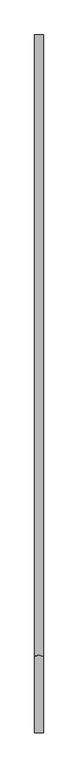
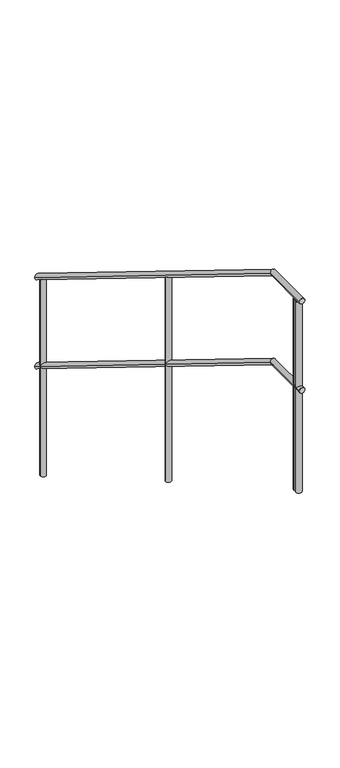
"""IFC4 building model written with IfcOpenShell, lengths in millimetres: railing geometry."""

from ifc_helpers import new_model, si_unit, point, frame, frame_2d, origin, place, context, project, spatial, circle_curve, ellipse_curve, trimmed, segment, composite_curve, outline, extrude, source, transform, mapped, element, save
from ifc_brep_helpers import plane_surface, cylinder_surface, advanced_brep


def railing_1ddb9561(model_context):
    return source(origin(), model_context, "Body", "SolidModel", [
        advanced_brep(
        [(-2206.0, 15342.7934796, -450.9609787), (-2176.0, 15342.7934796, -450.9609787), (-2176.0, 13178.5366941, 885.0), (-2206.0, 13178.5366941, 885.0), (-2206.0, 12912.7934796, 885.0), (-2176.0, 12912.7934796, 885.0)],
        [
            (0, 1, ellipse_curve(frame((-2191.0, 15342.7934796, -450.9609787), z_axis=(0.0, 1.0, 0.0), x_axis=(0.0, 0.0, -1.0)), 17.6276454, 15.0)),
            (1, 0, ellipse_curve(frame((-2191.0, 15342.7934796, -450.9609787), z_axis=(0.0, 1.0, 0.0), x_axis=(0.0, 0.0, -1.0)), 17.6276454, 15.0)),
            (1, 2),
            (2, 3, ellipse_curve(frame((-2191.0, 13178.5366941, 885.0), z_axis=(0.0, 0.9620125025549409, -0.27300539358770887), x_axis=(0.0, -0.27300539358770864, -0.962012502554941)), 15.5923129, 15.0)),
            (3, 0),
            (3, 2, ellipse_curve(frame((-2191.0, 13178.5366941, 885.0), z_axis=(0.0, 0.9620125025549409, -0.27300539358770887), x_axis=(0.0, -0.27300539358770864, -0.962012502554941)), 15.5923129, 15.0)),
            (4, 5, circle_curve(frame((-2191.0, 12912.7934796, 885.0), z_axis=(0.0, -1.0, 0.0), x_axis=(1.0, 0.0, 0.0)), 15.0)),
            (5, 4, circle_curve(frame((-2191.0, 12912.7934796, 885.0), z_axis=(0.0, -1.0, 0.0), x_axis=(1.0, 0.0, 0.0)), 15.0)),
            (2, 5),
            (4, 3),
        ],
        [
            plane_surface(frame((-2191.0, 15342.7934796, -433.3333333), z_axis=(0.0, 1.0, 0.0), x_axis=(0.0, 0.0, -1.0))),
            cylinder_surface(frame((-2191.0, 15334.9144415, -446.097375), z_axis=(0.0, 0.8509361101440404, -0.5252692037926169), x_axis=(1.0, 0.0, 0.0)), 15.0),
            plane_surface(frame((-2191.0, 12912.7934796, 900.0), z_axis=(0.0, -1.0, 0.0), x_axis=(0.0, 0.0, -1.0))),
            cylinder_surface(frame((-2191.0, 13182.7934796, 885.0), z_axis=(0.0, 1.0, 0.0), x_axis=(1.0, 0.0, 0.0)), 15.0),
        ],
        [
            (0, [[1, 2]]),
            (1, [[-2, 3, 4, 5]]),
            (1, [[-1, -5, 6, -3]]),
            (2, [[7, 8]]),
            (3, [[-4, 9, -7, 10]]),
            (3, [[-6, -10, -8, -9]]),
        ],
    ),
        advanced_brep(
        [(-2206.0, 15342.7934796, 49.0390213), (-2176.0, 15342.7934796, 49.0390213), (-2176.0, 13178.5366941, 1385.0), (-2206.0, 13178.5366941, 1385.0), (-2206.0, 12912.7934796, 1385.0), (-2176.0, 12912.7934796, 1385.0)],
        [
            (0, 1, ellipse_curve(frame((-2191.0, 15342.7934796, 49.0390213), z_axis=(0.0, 1.0, 0.0), x_axis=(0.0, 0.0, -1.0)), 17.6276454, 15.0)),
            (1, 0, ellipse_curve(frame((-2191.0, 15342.7934796, 49.0390213), z_axis=(0.0, 1.0, 0.0), x_axis=(0.0, 0.0, -1.0)), 17.6276454, 15.0)),
            (1, 2),
            (2, 3, ellipse_curve(frame((-2191.0, 13178.5366941, 1385.0), z_axis=(0.0, 0.9620125025549409, -0.27300539358770887), x_axis=(0.0, -0.27300539358770864, -0.962012502554941)), 15.5923129, 15.0)),
            (3, 0),
            (3, 2, ellipse_curve(frame((-2191.0, 13178.5366941, 1385.0), z_axis=(0.0, 0.9620125025549409, -0.27300539358770887), x_axis=(0.0, -0.27300539358770864, -0.962012502554941)), 15.5923129, 15.0)),
            (4, 5, circle_curve(frame((-2191.0, 12912.7934796, 1385.0), z_axis=(0.0, -1.0, 0.0), x_axis=(1.0, 0.0, 0.0)), 15.0)),
            (5, 4, circle_curve(frame((-2191.0, 12912.7934796, 1385.0), z_axis=(0.0, -1.0, 0.0), x_axis=(1.0, 0.0, 0.0)), 15.0)),
            (2, 5),
            (4, 3),
        ],
        [
            plane_surface(frame((-2191.0, 15342.7934796, 66.6666667), z_axis=(0.0, 1.0, 0.0), x_axis=(0.0, 0.0, -1.0))),
            cylinder_surface(frame((-2191.0, 15334.9144415, 53.902625), z_axis=(0.0, 0.8509361101440404, -0.5252692037926169), x_axis=(1.0, 0.0, 0.0)), 15.0),
            plane_surface(frame((-2191.0, 12912.7934796, 1400.0), z_axis=(0.0, -1.0, 0.0), x_axis=(0.0, 0.0, -1.0))),
            cylinder_surface(frame((-2191.0, 13182.7934796, 1385.0), z_axis=(0.0, 1.0, 0.0), x_axis=(1.0, 0.0, 0.0)), 15.0),
        ],
        [
            (0, [[1, 2]]),
            (1, [[-2, 3, 4, 5]]),
            (1, [[-1, -5, 6, -3]]),
            (2, [[7, 8]]),
            (3, [[-4, 9, -7, 10]]),
            (3, [[-6, -10, -8, -9]]),
        ],
    ),
        extrude(outline(composite_curve([segment(trimmed(circle_curve(frame_2d((-2191.0, 12942.7934796)), 15.0), [point((-2206.0, 12942.7934796))], [point((-2176.0, 12942.7934796))], False, "CARTESIAN"), True, "CONTINUOUS"), segment(trimmed(circle_curve(frame_2d((-2191.0, 12942.7934796)), 15.0), [point((-2176.0, 12942.7934796))], [point((-2206.0, 12942.7934796))], False, "CARTESIAN"), True, "CONTINUOUS")], self_intersect=False)), frame((0.0, 0.0, 300.0), z_axis=(0.0, 0.0, 1.0), x_axis=(1.0, 0.0, 0.0)), (0.0, 0.0, 1.0), 1070.0),
        advanced_brep(
        [(-2176.0, 14142.7934796, 777.4074074), (-2206.0, 14142.7934796, 777.4074074), (-2206.0, 14142.7934796, -366.6666667), (-2176.0, 14142.7934796, -366.6666667)],
        [
            (0, 1, ellipse_curve(frame((-2191.0, 14142.7934796, 777.4074074), z_axis=(0.0, -0.5252692037926167, -0.8509361101440406), x_axis=(0.0, -0.8509361101440406, 0.5252692037926162)), 17.6276454, 15.0)),
            (1, 2),
            (2, 3, circle_curve(frame((-2191.0, 14142.7934796, -366.6666667), z_axis=(0.0, 0.0, 1.0), x_axis=(-1.0, 0.0, 0.0)), 15.0)),
            (3, 0),
            (3, 2, circle_curve(frame((-2191.0, 14142.7934796, -366.6666667), z_axis=(0.0, 0.0, 1.0), x_axis=(-1.0, 0.0, 0.0)), 15.0)),
            (1, 0, ellipse_curve(frame((-2191.0, 14142.7934796, 777.4074074), z_axis=(0.0, -0.5252692037926167, -0.8509361101440406), x_axis=(0.0, -0.8509361101440406, 0.5252692037926162)), 17.6276454, 15.0)),
        ],
        [
            cylinder_surface(frame((-2191.0, 14142.7934796, -466.6666667), z_axis=(0.0, 0.0, 1.0), x_axis=(-1.0, 0.0, 0.0)), 15.0),
            plane_surface(frame((-2216.0, 14117.7934796, 792.8395062), z_axis=(0.0, 0.5252692037926167, 0.8509361101440406), x_axis=(1.0, 0.0, 0.0))),
            plane_surface(frame((-2216.0, 14167.7934796, -366.6666667), z_axis=(0.0, 0.0, -1.0), x_axis=(1.0, 0.0, 0.0))),
        ],
        [
            (0, [[1, 2, 3, 4]]),
            (0, [[5, -2, 6, -4]]),
            (1, [[-6, -1]]),
            (2, [[-5, -3]]),
        ],
    ),
        extrude(outline(composite_curve([segment(trimmed(circle_curve(frame_2d((-2191.0, 12962.7934796)), 15.0), [point((-2206.0, 12962.7934796))], [point((-2176.0, 12962.7934796))], False, "CARTESIAN"), True, "CONTINUOUS"), segment(trimmed(circle_curve(frame_2d((-2191.0, 12962.7934796)), 15.0), [point((-2176.0, 12962.7934796))], [point((-2206.0, 12962.7934796))], False, "CARTESIAN"), True, "CONTINUOUS")], self_intersect=False)), frame((0.0, 0.0, 300.0), z_axis=(0.0, 0.0, 1.0), x_axis=(1.0, 0.0, 0.0)), (0.0, 0.0, 1.0), 1070.0),
        advanced_brep(
        [(-2176.0, 15292.7934796, 67.5308642), (-2206.0, 15292.7934796, 67.5308642), (-2206.0, 15292.7934796, -1033.3333333), (-2176.0, 15292.7934796, -1033.3333333)],
        [
            (0, 1, ellipse_curve(frame((-2191.0, 15292.7934796, 67.5308642), z_axis=(0.0, -0.5252692037926167, -0.8509361101440406), x_axis=(0.0, -0.8509361101440406, 0.5252692037926162)), 17.6276454, 15.0)),
            (1, 2),
            (2, 3, circle_curve(frame((-2191.0, 15292.7934796, -1033.3333333), z_axis=(0.0, 0.0, 1.0), x_axis=(-1.0, 0.0, 0.0)), 15.0)),
            (3, 0),
            (3, 2, circle_curve(frame((-2191.0, 15292.7934796, -1033.3333333), z_axis=(0.0, 0.0, 1.0), x_axis=(-1.0, 0.0, 0.0)), 15.0)),
            (1, 0, ellipse_curve(frame((-2191.0, 15292.7934796, 67.5308642), z_axis=(0.0, -0.5252692037926167, -0.8509361101440406), x_axis=(0.0, -0.8509361101440406, 0.5252692037926162)), 17.6276454, 15.0)),
        ],
        [
            cylinder_surface(frame((-2191.0, 15292.7934796, -1133.3333333), z_axis=(0.0, 0.0, 1.0), x_axis=(-1.0, 0.0, 0.0)), 15.0),
            plane_surface(frame((-2216.0, 15267.7934796, 82.962963), z_axis=(0.0, 0.5252692037926167, 0.8509361101440406), x_axis=(1.0, 0.0, 0.0))),
            plane_surface(frame((-2216.0, 15317.7934796, -1033.3333333), z_axis=(0.0, 0.0, -1.0), x_axis=(1.0, 0.0, 0.0))),
        ],
        [
            (0, [[1, 2, 3, 4]]),
            (0, [[5, -2, 6, -4]]),
            (1, [[-6, -1]]),
            (2, [[-5, -3]]),
        ],
    ),
    ])


if __name__ == "__main__":
    model = new_model("IFC4")
    model_context = context("Model", 3, world=origin())
    ifc_project = project(units=[si_unit("LENGTHUNIT", "METRE", prefix="MILLI")], contexts=[model_context])
    site = spatial("IfcSite", under=ifc_project)
    building = spatial("IfcBuilding", under=site)
    placement = place(None, origin())
    railing_shape = railing_1ddb9561(model_context)
    element("IfcRailing", 1, at=placement, inside=building, context=model_context, shape_type="MappedRepresentation", body=[
        mapped(railing_shape, transform((0.0, 0.0, 0.0), x_axis=(1.0, 0.0, 0.0), y_axis=(0.0, 1.0, 0.0), z_axis=(0.0, 0.0, 1.0))),
    ])
    save(model, "model.ifc")
